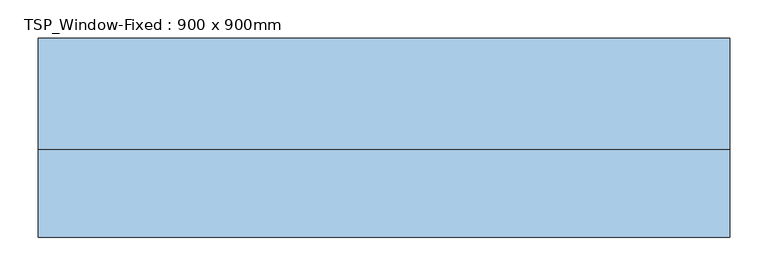
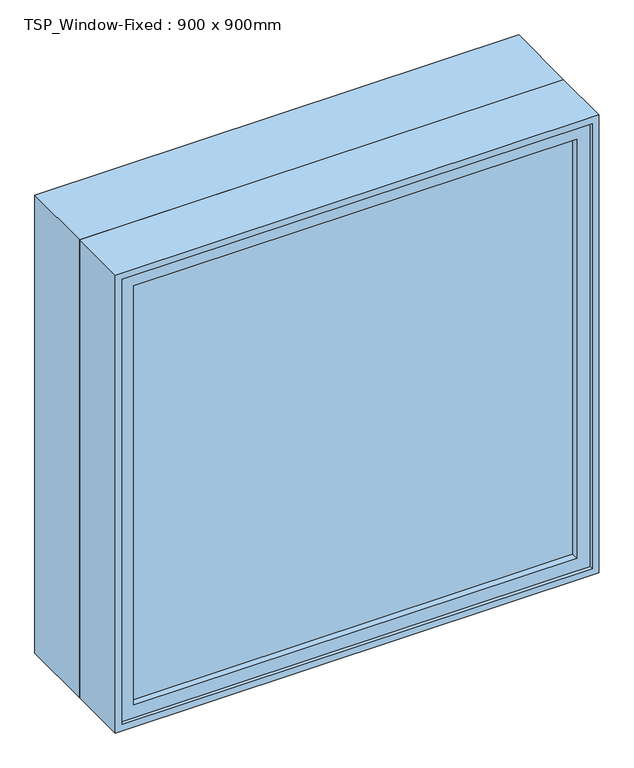
"""IFC4 building model written with IfcOpenShell, lengths in millimetres: window geometry, TSP_Window-Fixed : 900 x 900mm."""

from ifc_helpers import new_model, si_unit, frame, origin, place, context, project, spatial, polyline, outline, extrude, faceted_brep, source, transform, mapped, element, save


def tsp_window_fixed_900_x_900mm_656bd932(model_context):
    return source(origin(), model_context, "Body", "SolidModel", [
        faceted_brep([(450.0, -24.75, 1800.0), (-450.0, -24.75, 1800.0), (-450.0, -139.05, 1800.0), (450.0, -139.05, 1800.0), (-450.0, -24.75, 900.0), (-450.0, -139.05, 900.0), (450.0, -24.75, 900.0), (450.0, -139.05, 900.0), (418.25, -24.75, 1768.25), (-418.25, -24.75, 1768.25), (-418.25, -24.75, 931.75), (418.25, -24.75, 931.75), (-437.3, -139.05, 1787.3), (437.3, -139.05, 1787.3), (437.3, -139.05, 912.7), (-437.3, -139.05, 912.7), (418.25, -88.25, 1768.25), (-418.25, -88.25, 1768.25), (-437.3, -88.25, 1787.3), (437.3, -88.25, 1787.3), (-418.25, -88.25, 931.75), (-437.3, -88.25, 912.7), (418.25, -88.25, 931.75), (437.3, -88.25, 912.7)], [[[0, 1, 2, 3]], [[1, 4, 5, 2]], [[4, 6, 7, 5]], [[1, 0, 6, 4], [8, 9, 10, 11]], [[6, 0, 3, 7]], [[3, 2, 5, 7], [12, 13, 14, 15]], [[16, 17, 9, 8]], [[13, 12, 18, 19]], [[17, 20, 10, 9]], [[12, 15, 21, 18]], [[20, 22, 11, 10]], [[15, 14, 23, 21]], [[22, 16, 8, 11]], [[19, 18, 21, 23], [17, 16, 22, 20]], [[14, 13, 19, 23]]]),
        extrude(outline(polyline([(1800.0, -450.0), (900.0, -450.0), (900.0, 450.0), (1800.0, 450.0), (1800.0, -450.0)]), holes=[polyline([(1787.3, 437.3), (912.7, 437.3), (912.7, -437.3), (1787.3, -437.3), (1787.3, 437.3)])]), frame((0.0, -24.75, 0.0), z_axis=(0.0, 1.0, 0.0), x_axis=(0.0, 0.0, 1.0)), (0.0, 0.0, 1.0), 144.75),
        extrude(outline(polyline([(912.7, -437.3), (912.7, 437.3), (1787.3, 437.3), (1787.3, -437.3), (912.7, -437.3)]), holes=[polyline([(938.1, 411.9), (938.1, -411.9), (1761.9, -411.9), (1761.9, 411.9), (938.1, 411.9)])]), frame((0.0, -132.7, 0.0), z_axis=(0.0, 1.0, 0.0), x_axis=(0.0, 0.0, 1.0)), (0.0, 0.0, 1.0), 44.45),
        extrude(outline(polyline([(411.9, -120.0), (-411.9, -120.0), (-411.9, -113.65), (411.9, -113.65), (411.9, -120.0)])), frame((0.0, 0.0, 938.1), z_axis=(0.0, 0.0, 1.0), x_axis=(1.0, 0.0, 0.0)), (0.0, 0.0, 1.0), 823.8),
        extrude(outline(polyline([(-411.9, -100.95), (411.9, -100.95), (411.9, -107.3), (-411.9, -107.3), (-411.9, -100.95)])), frame((0.0, 0.0, 938.1), z_axis=(0.0, 0.0, 1.0), x_axis=(1.0, 0.0, 0.0)), (0.0, 0.0, 1.0), 823.8),
    ])


if __name__ == "__main__":
    model = new_model("IFC4")
    model_context = context("Model", 3, world=origin())
    ifc_project = project(units=[si_unit("LENGTHUNIT", "METRE", prefix="MILLI")], contexts=[model_context])
    site = spatial("IfcSite", under=ifc_project)
    building = spatial("IfcBuilding", under=site)
    placement = place(None, origin())
    tsp_window_fixed_900_x_900mm_shape = tsp_window_fixed_900_x_900mm_656bd932(model_context)
    element("IfcWindow", 1, ObjectType="TSP_Window-Fixed : 900 x 900mm", at=placement, inside=building, context=model_context, shape_type="MappedRepresentation", body=[
        mapped(tsp_window_fixed_900_x_900mm_shape, transform((0.0, 0.0, 0.0), x_axis=(1.0, 0.0, 0.0), y_axis=(0.0, 1.0, 0.0), z_axis=(0.0, 0.0, 1.0))),
    ])
    save(model, "model.ifc")

# Revit data of these elements
# Type "TSP_Window-Fixed : 900 x 900mm"
#   Type Mark = "HS 2412 F148"
#   Fire Rating = "0.5h"
#   Assembly Code = "B2020100"
#   Analytic Construction = "Double glazing - domestic"
#   Window Inset [instance default] = 0 mm
#   Wall Thickness [instance default] = 150 mm
#   Visual Light Transmittance = 0.81
#   Thermal Resistance (R) = 0.319569 (m²·K)/W
#   Solar Heat Gain Coefficient = 0.76
#   Rough Width = 915 mm
#   Rough Height = 915 mm
#   Interior Wall Closure [instance default] = 54.75 mm
#   Height = 900 mm
#   Heat Transfer Coefficient (U) = 3.12929 W/(m²·K)
#   Frame Extension [instance default] = 6.35 mm
#   Exterior Wall Closure [instance default] = 31.75 mm
#   Extension Jamb [instance default] = 54.75 mm
#   Default Sill Height = 900 mm
#   Width = 900 mm
#   Muntin Visibility = yes
#   Interior Trim Visibility [instance default] = yes
#   Exterior Trim Visibility [instance default] = yes
#   Extension Jamb Visibility [instance default] = yes
#   Interior Trim Material = Wood - Stained
#   Interior Frame Material = Wood - Stained
#   Glass Panel Material = Glass
#   Exterior Trim Material = Clad - White
#   Exterior Frame Material = Clad - White
#   Wall Closure = (empty or 0)
# Element 1 (IfcWindow, "TSP_Window-Fixed : 900 x 900mm")
#   Wall Thickness = 240 mm
#   Extension Jamb = 144.75 mm
#   Materials on its faces: "Wood - Stained", "Glass", "Clad - White"
# Materials
#   "Wood - Stained": class "Wood", colour RGB 224 178 126, transparency 0, Cost = 0
#   "Glass": class "Glass", colour RGB 0 128 192, transparency 0.9, Description = "Soda Lime Glass", Cost = 0
#   "Clad - White": class "Wood", colour RGB 242 242 238, transparency 0, Cost = 0
